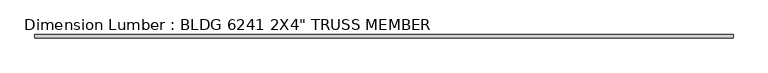
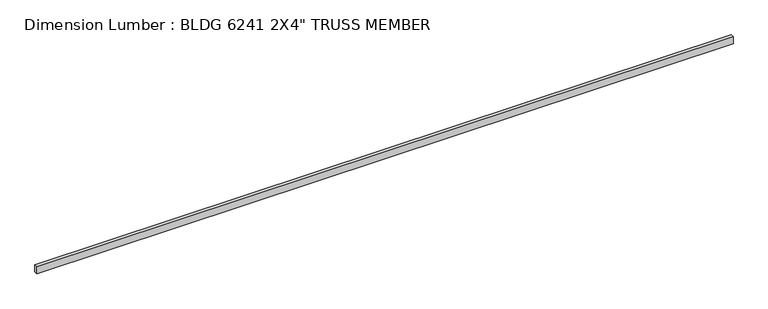
"""IFC4 building model written with IfcOpenShell, lengths in millimetres: beam geometry."""

import ifcopenshell
import ifcopenshell.guid

model = None  # the IFC model being written
_history = None  # IfcOwnerHistory: only IFC2X3 demands one
_inside = {}  # id of a spatial element -> (the spatial element, [elements in it])
_under = {}  # id of a project, library or spatial element -> (it, [spatial elements below it])
_declared = {}  # id of a project -> (the project, [libraries it declares])
_typed = {}  # id of a type object -> (the type object, [elements of that type])
_made_of = {}  # id of a material, layer set ... -> (it, [elements and type objects made of it])


def new_model(schema):
    """Start an empty IFC model of exactly this schema.

    Asked for "IFC4X3", IfcOpenShell would pick the latest addendum, in which some entities
    have other attributes; the version numbers below select the first issue.
    IFC2X3 requires an IfcOwnerHistory on every rooted entity: one is made here for all.
    """
    global model, _history
    if schema == "IFC4X3":
        model = ifcopenshell.file(schema_version=(4, 3, 0, 0))
    else:
        model = ifcopenshell.file(schema=schema)
    _inside.clear()
    _under.clear()
    _declared.clear()
    _typed.clear()
    _made_of.clear()
    _history = None
    if model.schema == "IFC2X3":
        org = make("IfcOrganization", Name="unknown")
        user = make(
            "IfcPersonAndOrganization",
            ThePerson=make("IfcPerson", FamilyName="unknown"),
            TheOrganization=org,
        )
        app = make(
            "IfcApplication",
            ApplicationDeveloper=org,
            Version="unknown",
            ApplicationFullName="unknown",
            ApplicationIdentifier="unknown",
        )
        _history = make(
            "IfcOwnerHistory",
            OwningUser=user,
            OwningApplication=app,
            ChangeAction="ADDED",
            CreationDate=0,
        )
    return model


def make(cls, **values):
    """One entity of the class cls with the attributes given. An attribute that is None is left unset."""
    return model.create_entity(
        cls, **{name: value for name, value in values.items() if value is not None}
    )


def rooted(cls, **values):
    """An entity with a GlobalId (a new one), such as an element, a storey or a relation."""
    return make(cls, GlobalId=ifcopenshell.guid.new(), OwnerHistory=_history, **values)


def si_unit(unit_type, name, prefix=None):
    """IfcSIUnit, for example si_unit("LENGTHUNIT", "METRE", prefix="MILLI")."""
    return make("IfcSIUnit", UnitType=unit_type, Prefix=prefix, Name=name)


def assignment(units):
    """IfcUnitAssignment: the units of a project."""
    return None if units is None else make("IfcUnitAssignment", Units=units)


def point(xyz):
    """IfcCartesianPoint."""
    return None if xyz is None else make("IfcCartesianPoint", Coordinates=xyz)


def direction(xyz):
    """IfcDirection."""
    return None if xyz is None else make("IfcDirection", DirectionRatios=xyz)


def frame(location, z_axis=None, x_axis=None):
    """IfcAxis2Placement3D, a coordinate frame: its origin and axes. An axis left out is left unset."""
    return make(
        "IfcAxis2Placement3D",
        Location=point(location),
        Axis=direction(z_axis),
        RefDirection=direction(x_axis),
    )


def origin():
    """The frame at (0, 0, 0) with its axes left unset."""
    return frame((0.0, 0.0, 0.0))


def place(relative_to, where):
    """IfcLocalPlacement: puts the frame where relative to a parent placement (None: the world)."""
    return make(
        "IfcLocalPlacement", PlacementRelTo=relative_to, RelativePlacement=where
    )


def context(
    kind, dimensions, precision=None, world=None, true_north=None, identifier=None
):
    """IfcGeometricRepresentationContext, for example the 3D "Model" context."""
    return make(
        "IfcGeometricRepresentationContext",
        ContextIdentifier=identifier,
        ContextType=kind,
        CoordinateSpaceDimension=dimensions,
        Precision=precision,
        WorldCoordinateSystem=world,
        TrueNorth=true_north,
    )


def project(units=None, contexts=None):
    """IfcProject with its units and contexts."""
    return rooted(
        "IfcProject",
        Name="project",
        RepresentationContexts=contexts,
        UnitsInContext=assignment(units),
    )


def spatial(cls, under=None, at=None, **own):
    """A site, building, storey or space (cls), placed at a placement, below another one or the project."""
    s = rooted(cls, ObjectPlacement=at, **own)
    if under is not None:
        _under.setdefault(under.id(), (under, []))[1].append(s)
    return s


def polyline(points):
    """IfcPolyline through the points."""
    return make("IfcPolyline", Points=[point(p) for p in points])


def outline(outer, holes=None, kind="AREA"):
    """IfcArbitraryClosedProfileDef: a profile drawn as a closed curve; with holes, ...WithVoids."""
    if holes is None:
        return make("IfcArbitraryClosedProfileDef", ProfileType=kind, OuterCurve=outer)
    return make(
        "IfcArbitraryProfileDefWithVoids",
        ProfileType=kind,
        OuterCurve=outer,
        InnerCurves=holes,
    )


def extrude(swept, where, along, depth):
    """IfcExtrudedAreaSolid: the profile swept, set in the frame where, extruded along a direction by depth."""
    return make(
        "IfcExtrudedAreaSolid",
        SweptArea=swept,
        Position=where,
        ExtrudedDirection=direction(along),
        Depth=depth,
    )


def shape(context_of_items, identifier, shape_type, items):
    """IfcShapeRepresentation: the items that make up one representation, for example the "Body"."""
    return make(
        "IfcShapeRepresentation",
        ContextOfItems=context_of_items,
        RepresentationIdentifier=identifier,
        RepresentationType=shape_type,
        Items=items,
    )


def source(mapping_origin, context_of_items, identifier, shape_type, items):
    """IfcRepresentationMap: a shape defined once, which mapped items show again and again."""
    return make(
        "IfcRepresentationMap",
        MappingOrigin=mapping_origin,
        MappedRepresentation=shape(context_of_items, identifier, shape_type, items),
    )


def transform(
    local_origin,
    x_axis=None,
    y_axis=None,
    z_axis=None,
    scale=None,
    scale2=None,
    scale3=None,
    uniform=True,
):
    """IfcCartesianTransformationOperator3D, or its non-uniform kind. x_axis, y_axis, z_axis: its Axis1, 2, 3."""
    if uniform:
        return make(
            "IfcCartesianTransformationOperator3D",
            Axis1=direction(x_axis),
            Axis2=direction(y_axis),
            LocalOrigin=point(local_origin),
            Scale=scale,
            Axis3=direction(z_axis),
        )
    return make(
        "IfcCartesianTransformationOperator3DnonUniform",
        Axis1=direction(x_axis),
        Axis2=direction(y_axis),
        LocalOrigin=point(local_origin),
        Scale=scale,
        Axis3=direction(z_axis),
        Scale2=scale2,
        Scale3=scale3,
    )


def mapped(mapping_source, mapping_target):
    """IfcMappedItem: shows the shape of a source again, moved by a transform."""
    return make(
        "IfcMappedItem", MappingSource=mapping_source, MappingTarget=mapping_target
    )


def made_of(thing, what):
    """Note that an element or type object is made of a material, layer set ...; save() writes the relation."""
    if what is not None:
        _made_of.setdefault(what.id(), (what, []))[1].append(thing)
    return thing


def element(
    cls,
    number,
    at=None,
    inside=None,
    cuts=None,
    type_object=None,
    material=None,
    context=None,
    identifier="Body",
    shape_type=None,
    held_by="IfcProductDefinitionShape",
    body=None,
    shapes=None,
    **own,
):
    """One element of the class cls, such as IfcWall. Its Tag is "e" and its number.

    at: its placement. inside: the storey or other place that contains it. cuts: it is an
    opening in that element (IfcRelVoidsElement). A single representation is given by context,
    identifier, shape_type and body (its items); several are given by shapes. held_by: the class
    of the entity that holds the representations. save() writes the other relations.
    """
    e = rooted(cls, Tag="e%d" % number, ObjectPlacement=at, **own)
    if body is not None:
        shapes = [shape(context, identifier, shape_type, body)]
    if shapes is not None:
        e.Representation = make(held_by, Representations=shapes)
    if inside is not None:
        _inside.setdefault(inside.id(), (inside, []))[1].append(e)
    if cuts is not None:
        rooted(
            "IfcRelVoidsElement", RelatingBuildingElement=cuts, RelatedOpeningElement=e
        )
    if type_object is not None:
        _typed.setdefault(type_object.id(), (type_object, []))[1].append(e)
    return made_of(e, material)


def aggregate(whole, parts):
    """IfcRelAggregates: a whole, such as a stair, and the parts it consists of."""
    return rooted("IfcRelAggregates", RelatingObject=whole, RelatedObjects=parts)


def save(model, path):
    """Write the relations noted so far, then the file.

    IfcRelAggregates (storeys below a building ...), IfcRelContainedInSpatialStructure (elements
    in a storey), IfcRelDefinesByType, IfcRelAssociatesMaterial and IfcRelDeclares: one each for
    every whole, place, type object, material and project.
    """
    for whole, parts in _under.values():
        aggregate(whole, parts)
    for where, things in _inside.values():
        rooted(
            "IfcRelContainedInSpatialStructure",
            RelatedElements=things,
            RelatingStructure=where,
        )
    for kind, things in _typed.values():
        rooted("IfcRelDefinesByType", RelatedObjects=things, RelatingType=kind)
    for what, things in _made_of.values():
        rooted("IfcRelAssociatesMaterial", RelatedObjects=things, RelatingMaterial=what)
    for by, libraries in _declared.values():
        rooted("IfcRelDeclares", RelatingContext=by, RelatedDefinitions=libraries)
    model.write(path)


def beam_8dd97a7c(model_context):
    return source(origin(), model_context, "Body", "SweptSolid", [
        extrude(outline(polyline([(5029.1999994, 25.4), (5029.1999994, -25.4), (-5029.1999994, -25.4), (-5029.1999994, 25.4), (5029.1999994, 25.4)])), frame((0.0, 0.0, -50.8), z_axis=(0.0, 0.0, 1.0), x_axis=(1.0, 0.0, 0.0)), (0.0, 0.0, 1.0), 101.6),
    ])


if __name__ == "__main__":
    model = new_model("IFC4")
    model_context = context("Model", 3, world=origin())
    ifc_project = project(units=[si_unit("LENGTHUNIT", "METRE", prefix="MILLI")], contexts=[model_context])
    site = spatial("IfcSite", under=ifc_project)
    building = spatial("IfcBuilding", under=site)
    placement = place(None, origin())
    beam_shape = beam_8dd97a7c(model_context)
    element("IfcBeam", 1, ObjectType="Dimension Lumber : BLDG 6241 2X4\" TRUSS MEMBER", at=placement, inside=building, context=model_context, shape_type="MappedRepresentation", body=[
        mapped(beam_shape, transform((0.0, 0.0, 0.0), x_axis=(1.0, 0.0, 0.0), y_axis=(0.0, 1.0, 0.0), z_axis=(0.0, 0.0, 1.0))),
    ])
    save(model, "model.ifc")

# Revit data of these elements
# Type "Dimension Lumber : BLDG 6241 2X4\" TRUSS MEMBER"
#   Assembly Code = "B10"
#   A = 0.273472 SF
#   Length [instance default] = 5' - 0"
#   b = 0' - 2"
#   d = 0' - 4"
#   Structural Material [instance default] = Softwood, Lumber
# Element 1 (IfcBeam, "Dimension Lumber : BLDG 6241 2X4\" TRUSS MEMBER")
#   Materials on its faces: "Softwood, Lumber"
# Materials
#   "Softwood, Lumber": class "Wood", colour RGB 223 192 134, transparency 0, Description = "Pinus Echinata", Cost = 0
